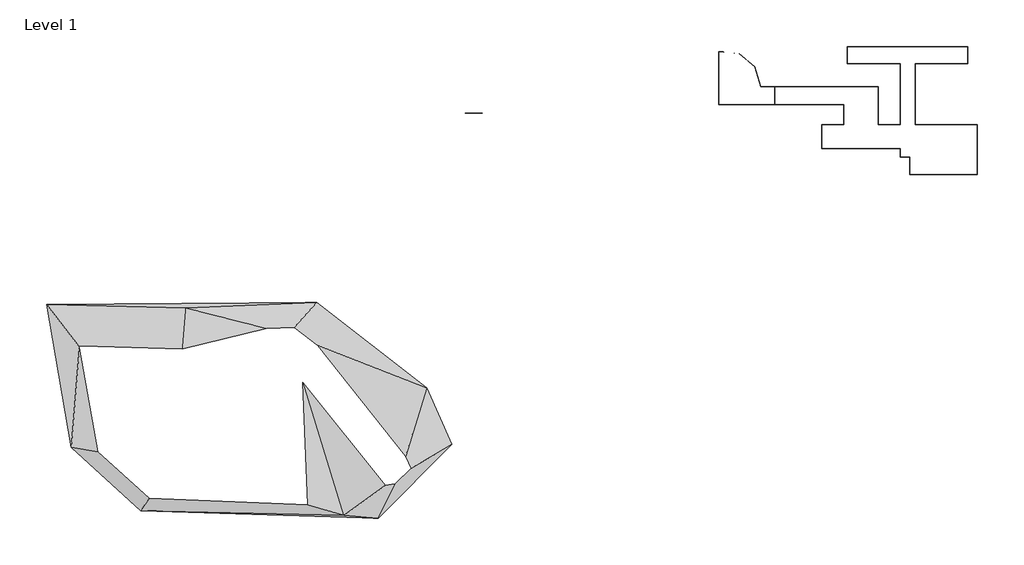
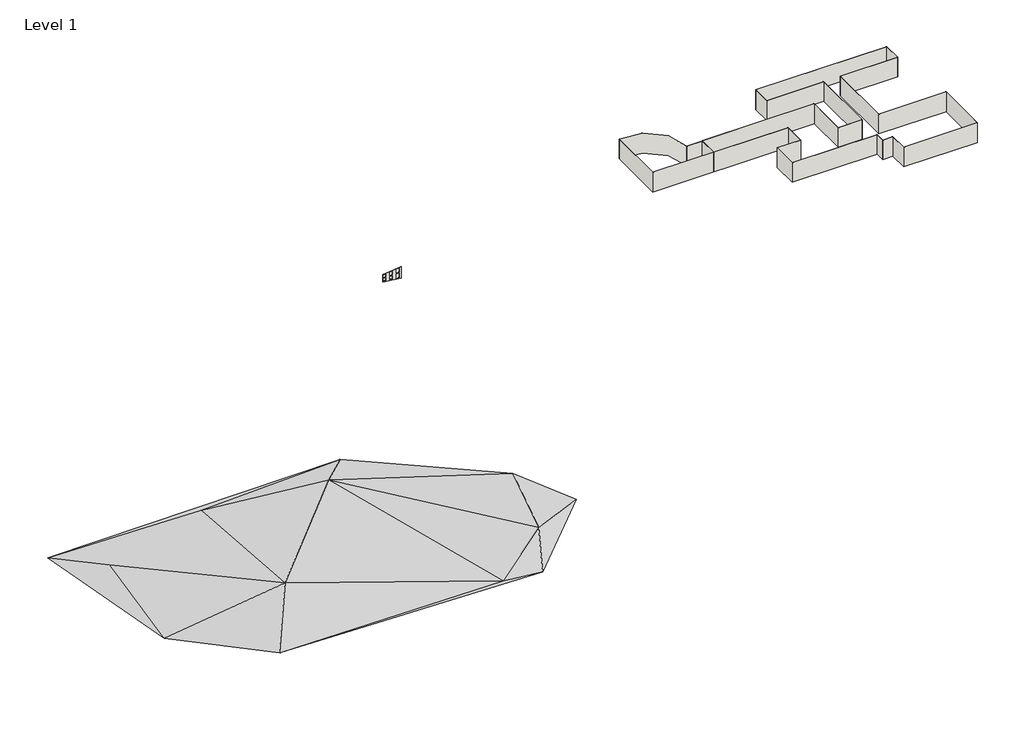
# One storey: 25 walls, 1 proxy.
"""IFC4 building model written with IfcOpenShell, lengths in millimetres."""

from ifc_helpers import new_model, si_unit, frame, origin, origin_with_axes, place, context, project, spatial, polyline, circle_curve, outline, extrude, faceted_brep, triangles, element, save
from ifc_brep_helpers import plane_surface, cylinder_surface, revolved_surface, advanced_brep

model = new_model("IFC4")

# Units and contexts
model_context = context("Model", 3, world=origin())
ifc_project = project(units=[si_unit("LENGTHUNIT", "METRE", prefix="MILLI")], contexts=[model_context])

# Site, building, storey
site = spatial("IfcSite", under=ifc_project)
building = spatial("IfcBuilding", under=site)
storey = spatial("IfcBuildingStorey", under=building, Name="Level 1", Elevation=0.0)

# Proxy
placement = place(None, origin())
element("IfcBuildingElementProxy", 1, Name="Building Element Proxy", at=placement, inside=storey, context=model_context, shape_type="Tessellation", body=[
    triangles([(-37088.1873413, -39186.9150513, 0.0), (-41143.7816528, -30119.489447, 0.0), (-58624.0263062, -16477.9546692, 0.0), (-79552.7813965, -17374.1639191, 0.0), (-101742.3572021, -16812.1261322, 0.0), (-97840.4186279, -39672.5784302, 0.0), (-86733.2640381, -49735.7269775, 0.0), (-48805.9930298, -50949.0994263, 0.0), (-45368.0307861, -43994.7146118, 1524.0), (-54350.1011353, -50494.8992432, 304.8), (-63213.9880005, -21539.5317627, 1524.0), (-81650.8765869, -42340.122583, 4572.0), (-96542.2094971, -23548.6812195, 1219.2)], [[6, 7, 12], [12, 7, 10], [6, 12, 13], [5, 13, 4], [13, 5, 6], [4, 13, 12], [5, 4, 3], [12, 11, 4], [10, 8, 9], [8, 10, 7], [9, 8, 1], [10, 9, 11], [11, 3, 4], [3, 11, 2], [2, 11, 9], [9, 1, 2], [10, 11, 12]], closed=False),
])

# Walls
element("IfcWall", 2, ObjectType="Generic - 8\"", at=placement, inside=storey, context=model_context, shape_type="Brep", body=[
    faceted_brep([(34367.5477784, 11846.8132666, 0.0), (34367.5477784, 21603.5882666, 0.0), (34367.5477784, 21603.5882666, 3048.0), (34367.5477784, 11846.8132666, 3048.0), (34364.3727784, 11846.8132666, 0.0), (34364.3727784, 11846.8132666, 3048.0), (34364.3727784, 11849.9882666, 3048.0), (34364.3727784, 21600.4132666, 3048.0), (34364.3727784, 21603.5882666, 3048.0), (34364.3727784, 21603.5882666, 0.0), (34364.3727784, 21600.4132666, 0.0), (34364.3727784, 11849.9882666, 0.0)], [[[0, 1, 2, 3]], [[4, 5, 6, 7, 8, 9, 10, 11]], [[1, 0, 4, 11, 10, 9]], [[3, 2, 8, 7, 6, 5]], [[2, 1, 9, 8]], [[0, 3, 5, 4]]]),
])
element("IfcWall", 3, ObjectType="Generic - 8\"", at=placement, inside=storey, context=model_context, shape_type="Brep", body=[
    faceted_brep([(36805.9477784, 11846.8132666, 0.0), (36805.9477784, 11849.9882666, 0.0), (36805.9477784, 21600.4132666, 0.0), (36805.9477784, 21603.5882666, 0.0), (36805.9477784, 21603.5882666, 3048.0), (36805.9477784, 21600.4132666, 3048.0), (36805.9477784, 11849.9882666, 3048.0), (36805.9477784, 11846.8132666, 3048.0), (36802.7727784, 11846.8132666, 0.0), (36802.7727784, 11846.8132666, 3048.0), (36802.7727784, 21603.5882666, 3048.0), (36802.7727784, 21603.5882666, 0.0)], [[[0, 1, 2, 3, 4, 5, 6, 7]], [[8, 9, 10, 11]], [[3, 2, 1, 0, 8, 11]], [[7, 6, 5, 4, 10, 9]], [[4, 3, 11, 10]], [[0, 7, 9, 8]]]),
])
element("IfcWall", 4, ObjectType="Generic - 8\"", at=placement, inside=storey, context=model_context, shape_type="Brep", body=[
    faceted_brep([(36805.9477784, 21600.4132666, 0.0), (45187.9477784, 21600.4132666, 0.0), (45187.9477784, 21600.4132666, 3048.0), (36805.9477784, 21600.4132666, 3048.0), (36805.9477784, 21603.5882666, 0.0), (36805.9477784, 21603.5882666, 3048.0), (45184.7727784, 21603.5882666, 3048.0), (45187.9477784, 21603.5882666, 3048.0), (45187.9477784, 21603.5882666, 0.0), (45184.7727784, 21603.5882666, 0.0)], [[[0, 1, 2, 3]], [[4, 5, 6, 7, 8, 9]], [[1, 0, 4, 9, 8]], [[3, 2, 7, 6, 5]], [[0, 3, 5, 4]], [[2, 1, 8, 7]]]),
])
element("IfcWall", 5, ObjectType="Generic - 8\"", at=placement, inside=storey, context=model_context, shape_type="Brep", body=[
    faceted_brep([(34364.3727784, 21603.5882666, 0.0), (25985.5477784, 21603.5882666, 0.0), (25982.3727784, 21603.5882666, 0.0), (25982.3727784, 21603.5882666, 3048.0), (25985.5477784, 21603.5882666, 3048.0), (34364.3727784, 21603.5882666, 3048.0), (34364.3727784, 21600.4132666, 0.0), (34364.3727784, 21600.4132666, 3048.0), (25982.3727784, 21600.4132666, 3048.0), (25982.3727784, 21600.4132666, 0.0)], [[[0, 1, 2, 3, 4, 5]], [[6, 7, 8, 9]], [[2, 1, 0, 6, 9]], [[5, 4, 3, 8, 7]], [[0, 5, 7, 6]], [[3, 2, 9, 8]]]),
])
element("IfcWall", 6, ObjectType="Generic - 8\"", at=placement, inside=storey, context=model_context, shape_type="Brep", body=[
    faceted_brep([(25982.3727784, 24343.6132666, 0.0), (25985.5477784, 24343.6132666, 0.0), (45184.7727784, 24343.6132666, 0.0), (45187.9477784, 24343.6132666, 0.0), (45187.9477784, 24343.6132666, 3048.0), (45184.7727784, 24343.6132666, 3048.0), (25985.5477784, 24343.6132666, 3048.0), (25982.3727784, 24343.6132666, 3048.0), (25982.3727784, 24346.7882666, 0.0), (25982.3727784, 24346.7882666, 3048.0), (45187.9477784, 24346.7882666, 3048.0), (45187.9477784, 24346.7882666, 0.0)], [[[0, 1, 2, 3, 4, 5, 6, 7]], [[8, 9, 10, 11]], [[3, 2, 1, 0, 8, 11]], [[7, 6, 5, 4, 10, 9]], [[4, 3, 11, 10]], [[0, 7, 9, 8]]]),
])
element("IfcWall", 7, ObjectType="Generic - 8\"", at=placement, inside=storey, context=model_context, shape_type="SweptSolid", body=[
    extrude(outline(polyline([(45187.9477784, 24343.6132666), (45187.9477784, 21603.5882666), (45184.7727784, 21603.5882666), (45184.7727784, 24343.6132666), (45187.9477784, 24343.6132666)])), origin_with_axes(), (0.0, 0.0, 1.0), 3048.0),
])
element("IfcWall", 8, ObjectType="Generic - 8\"", at=placement, inside=storey, context=model_context, shape_type="SweptSolid", body=[
    extrude(outline(polyline([(25985.5477784, 24343.6132666), (25985.5477784, 21603.5882666), (25982.3727784, 21603.5882666), (25982.3727784, 24343.6132666), (25985.5477784, 24343.6132666)])), origin_with_axes(), (0.0, 0.0, 1.0), 3048.0),
])
element("IfcWall", 9, ObjectType="Generic - 8\"", at=placement, inside=storey, context=model_context, shape_type="Brep", body=[
    faceted_brep([(36805.9477784, 11846.8132666, 0.0), (46708.7727784, 11846.8132666, 0.0), (46711.9477784, 11846.8132666, 0.0), (46711.9477784, 11846.8132666, 3048.0), (46708.7727784, 11846.8132666, 3048.0), (36805.9477784, 11846.8132666, 3048.0), (36805.9477784, 11849.9882666, 0.0), (36805.9477784, 11849.9882666, 3048.0), (46711.9477784, 11849.9882666, 3048.0), (46711.9477784, 11849.9882666, 0.0)], [[[0, 1, 2, 3, 4, 5]], [[6, 7, 8, 9]], [[2, 1, 0, 6, 9]], [[5, 4, 3, 8, 7]], [[0, 5, 7, 6]], [[3, 2, 9, 8]]]),
])
element("IfcWall", 10, ObjectType="Generic - 8\"", at=placement, inside=storey, context=model_context, shape_type="Brep", body=[
    faceted_brep([(46708.7727784, 11846.8132666, 0.0), (46708.7727784, 3925.1882666, 0.0), (46708.7727784, 3922.0132666, 0.0), (46708.7727784, 3922.0132666, 3048.0), (46708.7727784, 3925.1882666, 3048.0), (46708.7727784, 11846.8132666, 3048.0), (46711.9477784, 11846.8132666, 0.0), (46711.9477784, 11846.8132666, 3048.0), (46711.9477784, 3922.0132666, 3048.0), (46711.9477784, 3922.0132666, 0.0)], [[[0, 1, 2, 3, 4, 5]], [[6, 7, 8, 9]], [[2, 1, 0, 6, 9]], [[5, 4, 3, 8, 7]], [[0, 5, 7, 6]], [[3, 2, 9, 8]]]),
])
element("IfcWall", 11, ObjectType="Generic - 8\"", at=placement, inside=storey, context=model_context, shape_type="Brep", body=[
    faceted_brep([(46708.7727784, 3925.1882666, 0.0), (35891.5477784, 3925.1882666, 0.0), (35888.3727784, 3925.1882666, 0.0), (35888.3727784, 3925.1882666, 3048.0), (35891.5477784, 3925.1882666, 3048.0), (46708.7727784, 3925.1882666, 3048.0), (46708.7727784, 3922.0132666, 0.0), (46708.7727784, 3922.0132666, 3048.0), (35888.3727784, 3922.0132666, 3048.0), (35888.3727784, 3922.0132666, 0.0)], [[[0, 1, 2, 3, 4, 5]], [[6, 7, 8, 9]], [[2, 1, 0, 6, 9]], [[5, 4, 3, 8, 7]], [[0, 5, 7, 6]], [[3, 2, 9, 8]]]),
])
element("IfcWall", 12, ObjectType="Generic - 8\"", at=placement, inside=storey, context=model_context, shape_type="Brep", body=[
    faceted_brep([(35891.5477784, 3925.1882666, 0.0), (35891.5477784, 6668.3882666, 0.0), (35891.5477784, 6668.3882666, 3048.0), (35891.5477784, 3925.1882666, 3048.0), (35888.3727784, 3925.1882666, 0.0), (35888.3727784, 3925.1882666, 3048.0), (35888.3727784, 6665.2132666, 3048.0), (35888.3727784, 6668.3882666, 3048.0), (35888.3727784, 6668.3882666, 0.0), (35888.3727784, 6665.2132666, 0.0)], [[[0, 1, 2, 3]], [[4, 5, 6, 7, 8, 9]], [[1, 0, 4, 9, 8]], [[3, 2, 7, 6, 5]], [[0, 3, 5, 4]], [[2, 1, 8, 7]]]),
])
element("IfcWall", 13, ObjectType="Generic - 8\"", at=placement, inside=storey, context=model_context, shape_type="Brep", body=[
    faceted_brep([(35888.3727784, 6668.3882666, 0.0), (34367.5477784, 6668.3882666, 0.0), (34364.3727784, 6668.3882666, 0.0), (34364.3727784, 6668.3882666, 3048.0), (34367.5477784, 6668.3882666, 3048.0), (35888.3727784, 6668.3882666, 3048.0), (35888.3727784, 6665.2132666, 0.0), (35888.3727784, 6665.2132666, 3048.0), (34364.3727784, 6665.2132666, 3048.0), (34364.3727784, 6665.2132666, 0.0)], [[[0, 1, 2, 3, 4, 5]], [[6, 7, 8, 9]], [[2, 1, 0, 6, 9]], [[5, 4, 3, 8, 7]], [[0, 5, 7, 6]], [[3, 2, 9, 8]]]),
])
element("IfcWall", 14, ObjectType="Generic - 8\"", at=placement, inside=storey, context=model_context, shape_type="Brep", body=[
    faceted_brep([(34367.5477784, 6668.3882666, 0.0), (34367.5477784, 8039.9882666, 0.0), (34367.5477784, 8039.9882666, 3048.0), (34367.5477784, 6668.3882666, 3048.0), (34364.3727784, 6668.3882666, 0.0), (34364.3727784, 6668.3882666, 3048.0), (34364.3727784, 8036.8132666, 3048.0), (34364.3727784, 8039.9882666, 3048.0), (34364.3727784, 8039.9882666, 0.0), (34364.3727784, 8036.8132666, 0.0)], [[[0, 1, 2, 3]], [[4, 5, 6, 7, 8, 9]], [[1, 0, 4, 9, 8]], [[3, 2, 7, 6, 5]], [[0, 3, 5, 4]], [[2, 1, 8, 7]]]),
])
element("IfcWall", 15, ObjectType="Generic - 8\"", at=placement, inside=storey, context=model_context, shape_type="Brep", body=[
    faceted_brep([(34364.3727784, 8039.9882666, 0.0), (21870.7477784, 8039.9882666, 0.0), (21867.5727784, 8039.9882666, 0.0), (21867.5727784, 8039.9882666, 3048.0), (21870.7477784, 8039.9882666, 3048.0), (34364.3727784, 8039.9882666, 3048.0), (34364.3727784, 8036.8132666, 0.0), (34364.3727784, 8036.8132666, 3048.0), (21867.5727784, 8036.8132666, 3048.0), (21867.5727784, 8036.8132666, 0.0)], [[[0, 1, 2, 3, 4, 5]], [[6, 7, 8, 9]], [[2, 1, 0, 6, 9]], [[5, 4, 3, 8, 7]], [[0, 5, 7, 6]], [[3, 2, 9, 8]]]),
])
element("IfcWall", 16, ObjectType="Generic - 8\"", at=placement, inside=storey, context=model_context, shape_type="Brep", body=[
    faceted_brep([(21870.7477784, 8039.9882666, 0.0), (21870.7477784, 11846.8132666, 0.0), (21870.7477784, 11849.9882666, 0.0), (21870.7477784, 11849.9882666, 3048.0), (21870.7477784, 11846.8132666, 3048.0), (21870.7477784, 8039.9882666, 3048.0), (21867.5727784, 8039.9882666, 0.0), (21867.5727784, 8039.9882666, 3048.0), (21867.5727784, 11849.9882666, 3048.0), (21867.5727784, 11849.9882666, 0.0)], [[[0, 1, 2, 3, 4, 5]], [[6, 7, 8, 9]], [[2, 1, 0, 6, 9]], [[5, 4, 3, 8, 7]], [[0, 5, 7, 6]], [[3, 2, 9, 8]]]),
])
element("IfcWall", 17, ObjectType="Generic - 8\"", at=placement, inside=storey, context=model_context, shape_type="Brep", body=[
    faceted_brep([(21870.7477784, 11846.8132666, 0.0), (25375.9477784, 11846.8132666, 0.0), (25375.9477784, 11846.8132666, 3048.0), (21870.7477784, 11846.8132666, 3048.0), (21870.7477784, 11849.9882666, 0.0), (21870.7477784, 11849.9882666, 3048.0), (25372.7727784, 11849.9882666, 3048.0), (25375.9477784, 11849.9882666, 3048.0), (25375.9477784, 11849.9882666, 0.0), (25372.7727784, 11849.9882666, 0.0)], [[[0, 1, 2, 3]], [[4, 5, 6, 7, 8, 9]], [[1, 0, 4, 9, 8]], [[3, 2, 7, 6, 5]], [[0, 3, 5, 4]], [[2, 1, 8, 7]]]),
])
element("IfcWall", 18, ObjectType="Generic - 8\"", at=placement, inside=storey, context=model_context, shape_type="Brep", body=[
    faceted_brep([(25375.9477784, 11849.9882666, 0.0), (25375.9477784, 15050.3882666, 0.0), (25375.9477784, 15050.3882666, 3048.0), (25375.9477784, 11849.9882666, 3048.0), (25372.7727784, 11849.9882666, 0.0), (25372.7727784, 11849.9882666, 3048.0), (25372.7727784, 15047.2132666, 3048.0), (25372.7727784, 15050.3882666, 3048.0), (25372.7727784, 15050.3882666, 0.0), (25372.7727784, 15047.2132666, 0.0)], [[[0, 1, 2, 3]], [[4, 5, 6, 7, 8, 9]], [[1, 0, 4, 9, 8]], [[3, 2, 7, 6, 5]], [[0, 3, 5, 4]], [[2, 1, 8, 7]]]),
])
element("IfcWall", 19, ObjectType="Generic - 8\"", at=placement, inside=storey, context=model_context, shape_type="Brep", body=[
    faceted_brep([(25372.7727784, 15050.3882666, 0.0), (14403.1477784, 15050.3882666, 0.0), (14399.9727784, 15050.3882666, 0.0), (5462.6729099, 15050.3882666, 0.0), (5462.6729099, 15050.3882666, 3048.0), (14399.9727784, 15050.3882666, 3048.0), (14403.1477784, 15050.3882666, 3048.0), (25372.7727784, 15050.3882666, 3048.0), (25372.7727784, 15047.2132666, 0.0), (25372.7727784, 15047.2132666, 3048.0), (5462.6729099, 15047.2132666, 3048.0), (5462.6729099, 15047.2132666, 0.0)], [[[0, 1, 2, 3, 4, 5, 6, 7]], [[8, 9, 10, 11]], [[3, 2, 1, 0, 8, 11]], [[7, 6, 5, 4, 10, 9]], [[0, 7, 9, 8]], [[4, 3, 11, 10]]]),
])
element("IfcWall", 20, ObjectType="Generic - 8\"", at=placement, inside=storey, context=model_context, shape_type="Brep", body=[
    faceted_brep([(34364.3727784, 11849.9882666, 0.0), (30862.3477784, 11849.9882666, 0.0), (30859.1727784, 11849.9882666, 0.0), (30859.1727784, 11849.9882666, 3048.0), (30862.3477784, 11849.9882666, 3048.0), (34364.3727784, 11849.9882666, 3048.0), (34364.3727784, 11846.8132666, 0.0), (34364.3727784, 11846.8132666, 3048.0), (30859.1727784, 11846.8132666, 3048.0), (30859.1727784, 11846.8132666, 0.0)], [[[0, 1, 2, 3, 4, 5]], [[6, 7, 8, 9]], [[2, 1, 0, 6, 9]], [[5, 4, 3, 8, 7]], [[0, 5, 7, 6]], [[3, 2, 9, 8]]]),
])
element("IfcWall", 21, ObjectType="Generic - 8\"", at=placement, inside=storey, context=model_context, shape_type="Brep", body=[
    faceted_brep([(30862.3477784, 11849.9882666, 0.0), (30862.3477784, 17945.9882666, 0.0), (30862.3477784, 17945.9882666, 3048.0), (30862.3477784, 11849.9882666, 3048.0), (30859.1727784, 11849.9882666, 0.0), (30859.1727784, 11849.9882666, 3048.0), (30859.1727784, 17942.8132666, 3048.0), (30859.1727784, 17945.9882666, 3048.0), (30859.1727784, 17945.9882666, 0.0), (30859.1727784, 17942.8132666, 0.0)], [[[0, 1, 2, 3]], [[4, 5, 6, 7, 8, 9]], [[1, 0, 4, 9, 8]], [[3, 2, 7, 6, 5]], [[0, 3, 5, 4]], [[2, 1, 8, 7]]]),
])
element("IfcWall", 22, ObjectType="Generic - 8\"", at=placement, inside=storey, context=model_context, shape_type="AdvancedBrep", body=[
    advanced_brep(
    [(30859.1727784, 17945.9882666, 0.0), (12117.1738942, 17945.9882666, 0.0), (12113.9984787, 17945.9882666, 0.0), (12113.9984787, 17945.9882666, 3048.0), (12117.1738942, 17945.9882666, 3048.0), (30859.1727784, 17945.9882666, 3048.0), (30859.1727784, 17942.8132666, 0.0), (30859.1727784, 17942.8132666, 3048.0), (14403.1477784, 17942.8132666, 3048.0), (14399.9727784, 17942.8132666, 3048.0), (12113.9461968, 17942.8132666, 3048.0), (12113.9461968, 17942.8132666, 0.0), (14399.9727784, 17942.8132666, 0.0), (14403.1477784, 17942.8132666, 0.0)],
    [
        (0, 1),
        (1, 2),
        (2, 3),
        (3, 4),
        (4, 5),
        (5, 0),
        (6, 7),
        (7, 8),
        (8, 9),
        (9, 10),
        (10, 11),
        (11, 12),
        (12, 13),
        (13, 6),
        (0, 6),
        (11, 2, circle_curve(frame((6522.9072992, 18036.4673562, 0.0), z_axis=(0.0, 0.0, 1.0), x_axis=(1.0, 0.0, 0.0)), 5591.8232307)),
        (3, 10, circle_curve(frame((6522.9072992, 18036.4673562, 3048.0), z_axis=(0.0, 0.0, -1.0), x_axis=(1.0, 0.0, 0.0)), 5591.8232307)),
        (7, 5),
    ],
    [
        plane_surface(frame((30860.7602784, 17945.9882666, 0.0), z_axis=(0.0, 1.0, 0.0), x_axis=(-1.0, 0.0, 0.0))),
        plane_surface(frame((30860.7602784, 17942.8132666, 0.0), z_axis=(0.0, -1.0, 0.0), x_axis=(1.0, 0.0, 0.0))),
        plane_surface(frame((30860.7602784, 17945.9882666, 0.0), z_axis=(0.0, 0.0, -1.0), x_axis=(0.0, -1.0, 0.0))),
        plane_surface(frame((12115.5602784, 17945.9882666, 3048.0), z_axis=(0.0, 0.0, 1.0), x_axis=(0.0, -1.0, 0.0))),
        plane_surface(frame((30859.1727784, 11848.4007666, 0.0), z_axis=(1.0, 0.0, 0.0), x_axis=(0.0, -1.0, 0.0))),
        revolved_surface(polyline([(12114.7305299, 18036.4673562, 0.0), (12114.7305299, 18036.4673562, 3048.0)]), (6522.9072992, 18036.4673562, 0.0), (0.0, 0.0, -1.0)),
    ],
    [
        (0, [[1, 2, 3, 4, 5, 6]]),
        (1, [[7, 8, 9, 10, 11, 12, 13, 14]]),
        (2, [[-2, -1, 15, -14, -13, -12, 16]]),
        (3, [[-5, -4, 17, -10, -9, -8, 18]]),
        (4, [[-6, -18, -7, -15]]),
        (5, [[-3, -16, -11, -17]]),
    ],
),
])
element("IfcWall", 23, ObjectType="Generic - 8\"", at=placement, inside=storey, context=model_context, shape_type="AdvancedBrep", body=[
    advanced_brep(
    [(5459.4979099, 23526.2439923, 3048.0), (5462.6751985, 23526.8584204, 3048.0), (12113.9984787, 17945.9882666, 3048.0), (12117.1738942, 17945.9882666, 3048.0), (5459.4979099, 23529.4779763, 3048.0), (5459.4979099, 23526.2439923, 0.0), (5459.4979099, 23529.4779763, 0.0), (12117.1738942, 17945.9882666, 0.0), (12113.9984787, 17945.9882666, 0.0), (5462.6751985, 23526.8584204, 0.0)],
    [
        (0, 1, circle_curve(frame((6522.9072992, 18036.4673562, 3048.0), z_axis=(0.0, 0.0, -1.0), x_axis=(1.0, 0.0, 0.0)), 5591.8232307)),
        (1, 2, circle_curve(frame((6522.9072992, 18036.4673562, 3048.0), z_axis=(0.0, 0.0, -1.0), x_axis=(1.0, 0.0, 0.0)), 5591.8231504)),
        (2, 3),
        (3, 4, circle_curve(frame((6522.9072992, 18036.4673562, 3048.0), z_axis=(0.0, 0.0, 1.0), x_axis=(1.0, 0.0, 0.0)), 5594.9982307)),
        (4, 0),
        (5, 6),
        (6, 7, circle_curve(frame((6522.9072992, 18036.4673562, 0.0), z_axis=(0.0, 0.0, -1.0), x_axis=(1.0, 0.0, 0.0)), 5594.9982307)),
        (7, 8),
        (8, 9, circle_curve(frame((6522.9072992, 18036.4673562, 0.0), z_axis=(0.0, 0.0, 1.0), x_axis=(1.0, 0.0, 0.0)), 5591.8232307)),
        (9, 5, circle_curve(frame((6522.9072992, 18036.4673562, 0.0), z_axis=(0.0, 0.0, 1.0), x_axis=(1.0, 0.0, 0.0)), 5591.8231504)),
        (0, 5),
        (8, 2),
        (3, 7),
        (6, 4),
    ],
    [
        plane_surface(frame((12114.7305299, 18036.4673562, 3048.0), z_axis=(0.0, 0.0, 1.0), x_axis=(0.0, -1.0, 0.0))),
        plane_surface(frame((12114.7305299, 18036.4673562, 0.0), z_axis=(0.0, 0.0, -1.0), x_axis=(0.0, 1.0, 0.0))),
        revolved_surface(polyline([(12114.7305299, 18036.4673562, 0.0), (12114.7305299, 18036.4673562, 3048.0)]), (6522.9072992, 18036.4673562, 0.0), (0.0, 0.0, -1.0)),
        cylinder_surface(frame((6522.9072992, 18036.4673562, 0.0), z_axis=(0.0, 0.0, 1.0), x_axis=(1.0, 0.0, 0.0)), 5594.9982307),
        plane_surface(frame((30860.7602784, 17945.9882666, 0.0), z_axis=(0.0, -1.0, 0.0), x_axis=(-1.0, 0.0, 0.0))),
        plane_surface(frame((5459.4979099, 23528.1681745, 0.0), z_axis=(-1.0, 0.0, 0.0), x_axis=(0.0, -1.0, 0.0))),
    ],
    [
        (0, [[1, 2, 3, 4, 5]]),
        (1, [[6, 7, 8, 9, 10]]),
        (2, [[-2, -1, 11, -10, -9, 12]]),
        (3, [[-4, 13, -7, 14]]),
        (4, [[-3, -12, -8, -13]]),
        (5, [[-5, -14, -6, -11]]),
    ],
),
])
element("IfcWall", 24, ObjectType="Generic - 8\"", at=placement, inside=storey, context=model_context, shape_type="AdvancedBrep", body=[
    advanced_brep(
    [(5459.4979099, 23526.2439923, 0.0), (5459.4979099, 15047.2132666, 0.0), (5459.4979099, 15047.2132666, 3048.0), (5459.4979099, 23526.2439923, 3048.0), (5462.6729099, 23526.8580602, 0.0), (5462.6729099, 23526.8580602, 3048.0), (5462.6729099, 15050.3882666, 3048.0), (5462.6729099, 15047.2132666, 3048.0), (5462.6729099, 15047.2132666, 0.0), (5462.6729099, 15050.3882666, 0.0)],
    [
        (0, 1),
        (1, 2),
        (2, 3),
        (3, 0),
        (4, 5),
        (5, 6),
        (6, 7),
        (7, 8),
        (8, 9),
        (9, 4),
        (0, 4, circle_curve(frame((6522.9072992, 18036.4673562, 0.0), z_axis=(0.0, 0.0, -1.0), x_axis=(1.0, 0.0, 0.0)), 5591.8232307)),
        (8, 1),
        (2, 7),
        (5, 3, circle_curve(frame((6522.9072992, 18036.4673562, 3048.0), z_axis=(0.0, 0.0, 1.0), x_axis=(1.0, 0.0, 0.0)), 5591.8232307)),
    ],
    [
        plane_surface(frame((5459.4979099, 23528.1681745, 0.0), z_axis=(-1.0, 0.0, 0.0), x_axis=(0.0, -1.0, 0.0))),
        plane_surface(frame((5462.6729099, 23528.1681745, 0.0), z_axis=(1.0, 0.0, 0.0), x_axis=(0.0, 1.0, 0.0))),
        plane_surface(frame((5459.4979099, 23528.1681745, 0.0), z_axis=(0.0, 0.0, -1.0), x_axis=(1.0, 0.0, 0.0))),
        plane_surface(frame((5459.4979099, 15048.8007666, 3048.0), z_axis=(0.0, 0.0, 1.0), x_axis=(1.0, 0.0, 0.0))),
        cylinder_surface(frame((6522.9072992, 18036.4673562, 0.0), z_axis=(0.0, 0.0, -1.0), x_axis=(1.0, 0.0, 0.0)), 5591.8232307),
        plane_surface(frame((25374.3602784, 15047.2132666, 0.0), z_axis=(0.0, -1.0, 0.0), x_axis=(1.0, 0.0, 0.0))),
    ],
    [
        (0, [[1, 2, 3, 4]]),
        (1, [[5, 6, 7, 8, 9, 10]]),
        (2, [[-1, 11, -10, -9, 12]]),
        (3, [[-3, 13, -7, -6, 14]]),
        (4, [[-4, -14, -5, -11]]),
        (5, [[-2, -12, -8, -13]]),
    ],
),
])
element("IfcWall", 25, ObjectType="Generic - 8\"", at=placement, inside=storey, context=model_context, shape_type="SweptSolid", body=[
    extrude(outline(polyline([(954.90746, -34959.3167896), (669.6657188, -32245.4229055), (2455.079747, -32245.4229055), (2169.8380057, -34959.3167896), (954.90746, -34959.3167896)]), holes=[polyline([(1494.090381, -34857.7167896), (1494.090381, -34530.0213791), (1053.2482054, -34530.0213791), (1087.690381, -34857.7167896), (1494.090381, -34857.7167896)]), polyline([(1494.090381, -33950.830558), (1494.090381, -33546.9351474), (943.6392627, -33546.9351474), (986.090381, -33950.830558), (1494.090381, -33950.830558)]), polyline([(1494.090381, -32998.1528292), (1494.090381, -32518.0574186), (788.5696151, -32518.0574186), (839.0296761, -32998.1528292), (1494.090381, -32998.1528292)]), polyline([(2054.5766603, -34857.7167896), (2089.0188358, -34530.0213791), (1648.1766603, -34530.0213791), (1648.1766603, -34857.7167896), (2054.5766603, -34857.7167896)]), polyline([(2156.1766603, -33950.830558), (2198.6277786, -33546.9351474), (1648.1766603, -33546.9351474), (1648.1766603, -33950.830558), (2156.1766603, -33950.830558)]), polyline([(2277.8373652, -32998.1528292), (2328.2974261, -32518.0574186), (1648.1766603, -32518.0574186), (1648.1766603, -32998.1528292), (2277.8373652, -32998.1528292)])]), frame((0.0, 13708.044474, 0.0), z_axis=(0.0, 1.0, 0.0), x_axis=(0.0, 0.0, 1.0)), (0.0, 0.0, 1.0), 3.175),
])
element("IfcWall", 26, ObjectType="Generic - 8\"", at=placement, inside=storey, context=model_context, shape_type="SweptSolid", body=[
    extrude(outline(polyline([(14399.9727784, 15050.3882666), (14399.9727784, 17942.8132666), (14403.1477784, 17942.8132666), (14403.1477784, 15050.3882666), (14399.9727784, 15050.3882666)])), origin_with_axes(), (0.0, 0.0, 1.0), 3048.0),
])

save(model, "model.ifc")

# Revit data of these elements
# Project information
#   Project Issue Date = "Issue Date"
#   Project Status = "Project Status"
#   Client Name = "Owner"
#   Project Address = "Enter address here"
#   Project Name = "Project Name"
#   Project Number = "Project Number"
# Type "Generic - 8\""
#   Assembly Code = "B2010"
#   Layers, outside or top first: 0' - 0 1/8" no material (function 1)
# Element 1 (IfcBuildingElementProxy)
#   Material = none
#   Phase Created = Project Completion
# Elements 2, 3, 4, 5, 6, 7, 8, 9, 10, 11, 12, 13, 14, 15, 16, 17, 18, 19, 20, 21, 22, 24, 25, 26 (IfcWall, "Generic - 8\"")
#   Top Offset = 0' - 0"
#   Base Offset = 0' - 0"
#   wall height = 10' - 0"
#   Phase Created = Project Completion
#   Base Constraint = Level 1
#   Top Constraint = Level 2
#   Materials on its faces: "Default Wall"
# Element 23 (IfcWall, "Generic - 8\"")
#   Top Offset = 0' - 0"
#   Base Offset = 0' - 0"
#   Unconnected Height = 20' - 0"
#   wall height = 10' - 0"
#   Phase Created = Project Completion
#   Materials on its faces: "Default Wall"
# Materials
#   "Default Wall": class "Miscellaneous", colour RGB 128 128 128, transparency 0, Cost = 0
# Space at (8928.517, 18846.425) mm, phase "Project Completion", upper level "Level 1", upper offset 10' - 0", lower offset 0' - 0"
#   Number = "1"
#   Name = "Space"
#   Actual Lighting Load per area = 0
#   Actual Power Load per area = 0
#   Sensible Heat Gain per person = 0
#   Specified Lighting Load = 6595.38 (stored number, unit not read)
#   Specified Power Load = 8574 (stored number, unit not read)
#   Latent Heat Gain per person = 0
#   Total Heat Gain per person = 0
#   Area per Person = 0
#   Number of People = 1.99236 (stored number, unit not read)
#   Lighting Load Units = 0
#   Power Load Units = 0
#   Return Airflow = 0
#   Occupancy Unit = -1
#   Condition Type = 2
#   Construction Type = none
